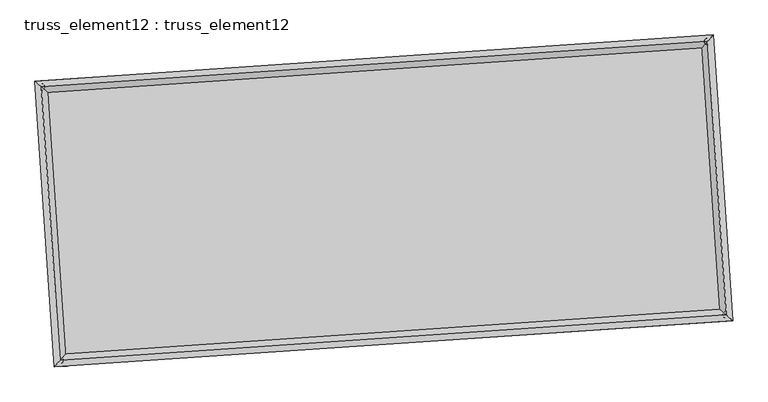
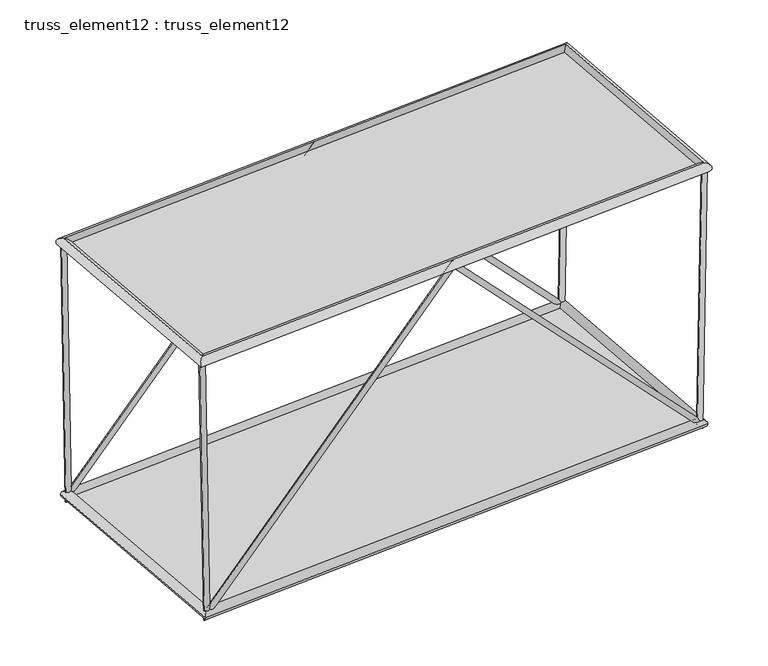
"""IFC4 building model written with IfcOpenShell, lengths in millimetres: plate geometry, truss_element12 : truss_element12."""

from ifc_helpers import new_model, si_unit, frame, origin, origin_with_axes, place, context, project, spatial, polyline, circle_curve, ellipse_curve, outline, extrude, source, transform, mapped, element, save
from ifc_brep_helpers import plane_surface, cylinder_surface, advanced_brep


def truss_element12_truss_element12_eb7cdb9d(model_context):
    return source(origin(), model_context, "Body", "SolidModel", [
        advanced_brep(
        [(-3751.912515, 2270.2937696, 5000.1099238), (-3851.0007491, 2256.9335317, 4998.3704092), (-3667.056332, 2276.0797902, 121.9949924), (-3761.9305509, 2263.0068899, -121.9949924), (1063.0047993, 2598.6046781, 5071.3707935), (1063.4636729, 2592.032179, 4927.1341285), (5794.4609613, 2921.2246878, 122.0048162), (5890.3000157, 2921.1558007, -122.0048162), (5877.9325391, 2926.9162974, 5000.120325), (5977.9176694, 2927.1301154, 4998.409186)],
        [
            (0, 1, circle_curve(frame((-3801.4566321, 2263.6136507, 4999.2401665), z_axis=(-0.017392638132463133, -0.0011859378786482353, 0.9998480332981313), x_axis=(-0.13360270549459097, 0.9910343071078557, -0.0011485729311865587)), 50.0)),
            (1, 0, circle_curve(frame((-3801.4566321, 2263.6136507, 4999.2401665), z_axis=(-0.017392638132463133, -0.0011859378786482353, 0.9998480332981313), x_axis=(-0.13360270549459097, 0.9910343071078557, -0.0011485729311865587)), 50.0)),
            (0, 2),
            (2, 3, ellipse_curve(frame((-3714.4934414, 2269.54334, 0.0), z_axis=(-0.9289957394028403, -0.06334468802646137, 0.36462908094418417), x_axis=(0.36378437978405503, 0.024805073983579777, 0.9311528517541036)), 131.300287, 50.0)),
            (3, 1),
            (3, 2, ellipse_curve(frame((-3714.4934414, 2269.54334, 0.0), z_axis=(-0.9289957394028403, -0.06334468802646137, 0.36462908094418417), x_axis=(0.36378437978405503, 0.024805073983579777, 0.9311528517541036)), 131.300287, 50.0)),
            (2, 4),
            (4, 5, ellipse_curve(frame((1063.2342361, 2595.3184285, 4999.252461), z_axis=(-0.9976833933321773, -0.06802823804168447, -7.414941499554083e-05), x_axis=(7.397764016911895e-05, 5.044254070666447e-06, -0.9999999972509321)), 72.2753704, 50.0)),
            (5, 3),
            (5, 4, ellipse_curve(frame((1063.2342361, 2595.3184285, 4999.252461), z_axis=(-0.9976833933321773, -0.06802823804168447, -7.414941499554083e-05), x_axis=(7.397764016911895e-05, 5.044254070666447e-06, -0.9999999972509321)), 72.2753704, 50.0)),
            (4, 6),
            (6, 7, ellipse_curve(frame((5842.3804885, 2921.1902443, 0.0), z_axis=(-0.9289170101606304, -0.06333931977871081, -0.36483053436384116), x_axis=(-0.36398536651592867, -0.02481877850480949, 0.9310739397039283)), 131.3219892, 50.0)),
            (7, 5),
            (7, 6, ellipse_curve(frame((5842.3804885, 2921.1902443, 0.0), z_axis=(-0.9289170101606304, -0.06333931977871081, -0.36483053436384116), x_axis=(-0.36398536651592867, -0.02481877850480949, 0.9310739397039283)), 131.3219892, 50.0)),
            (8, 9, circle_curve(frame((5927.9251043, 2927.0232064, 4999.2647555), z_axis=(0.017108923152044243, 0.001166592432629323, 0.9998529510936464), x_axis=(-0.002157828250047212, 0.9999970336184036, -0.001129836995660202)), 50.0)),
            (9, 8, circle_curve(frame((5927.9251043, 2927.0232064, 4999.2647555), z_axis=(0.017108923152044243, 0.001166592432629323, 0.9998529510936464), x_axis=(-0.002157828250047212, 0.9999970336184036, -0.001129836995660202)), 50.0)),
            (6, 8),
            (9, 7),
        ],
        [
            plane_surface(frame((-3801.4566321, 2313.6136155, 4999.2994724), z_axis=(-0.017392638132462068, -0.0011859378786532565, 0.9998480332981314), x_axis=(0.9998487366290929, -2.0629708890496073e-05, 0.017392625897830513))),
            cylinder_surface(frame((-3801.4566321, 2263.6136507, 4999.2401665), z_axis=(-0.017392638132463136, -0.0011859378786482355, 0.9998480332981315), x_axis=(-0.13360270549459097, 0.9910343071078557, -0.0011485729311865587)), 50.0),
            cylinder_surface(frame((-3714.4934414, 2269.54334, 0.0), z_axis=(-0.6901425550207472, -0.04705819734940098, -0.7221418003492527), x_axis=(-0.020412411512224723, 0.9987523229779233, -0.045575550489902014)), 50.0),
            cylinder_surface(frame((1063.2342361, 2595.3184285, 4999.252461), z_axis=(-0.6902493921239737, -0.047065482165348276, 0.7220392074264583), x_axis=(-0.11534170182495504, 0.9922794555315144, -0.045582605785589675)), 50.0),
            plane_surface(frame((5927.9251043, 2877.0232404, 4999.3230936), z_axis=(0.017108923152043723, 0.0011665924326239086, 0.9998529510936466), x_axis=(0.9998536316624437, -1.9962062093981113e-05, -0.017108911506539936))),
            cylinder_surface(frame((5842.3804885, 2921.1902443, 0.0), z_axis=(-0.017108923152044243, -0.001166592432629323, -0.9998529510936464), x_axis=(-0.002157828250047212, 0.9999970336184036, -0.001129836995660202)), 50.0),
        ],
        [
            (0, [[1, 2]]),
            (1, [[-1, 3, 4, 5]]),
            (1, [[-2, -5, 6, -3]]),
            (2, [[-4, 7, 8, 9]]),
            (2, [[-6, -9, 10, -7]]),
            (3, [[-8, 11, 12, 13]]),
            (3, [[-10, -13, 14, -11]]),
            (4, [[15, 16]]),
            (5, [[-12, 17, -16, 18]]),
            (5, [[-14, -18, -15, -17]]),
        ],
    ),
        advanced_brep(
        [(-3479.7995621, -1720.4398147, 5000.1099238), (-3578.8877962, -1733.8000526, 4998.3704092), (-3394.943379, -1714.6537941, 121.9949924), (-3489.817598, -1727.7266944, -121.9949924), (1335.1177522, -1392.1289062, 5071.3707935), (1335.5766258, -1398.7014053, 4927.1341285), (6066.5739142, -1069.5088965, 122.0048162), (6162.4129686, -1069.5777836, -122.0048162), (6150.045492, -1063.8172869, 5000.120325), (6250.0306223, -1063.6034689, 4998.409186)],
        [
            (0, 1, circle_curve(frame((-3529.3436792, -1727.1199336, 4999.2401665), z_axis=(-0.017392638132463636, -0.0011859378786482945, 0.9998480332981314), x_axis=(-0.1336027054945913, 0.9910343071078556, -0.0011485729311865723)), 50.0)),
            (1, 0, circle_curve(frame((-3529.3436792, -1727.1199336, 4999.2401665), z_axis=(-0.017392638132463636, -0.0011859378786482945, 0.9998480332981314), x_axis=(-0.1336027054945913, 0.9910343071078556, -0.0011485729311865723)), 50.0)),
            (0, 2),
            (2, 3, ellipse_curve(frame((-3442.3804885, -1721.1902443, 0.0), z_axis=(-0.9289957394028405, -0.06334468802646162, 0.3646290809441836), x_axis=(0.3637843797840544, 0.0248050739835798, 0.9311528517541038)), 131.300287, 50.0)),
            (3, 1),
            (3, 2, ellipse_curve(frame((-3442.3804885, -1721.1902443, 0.0), z_axis=(-0.9289957394028405, -0.06334468802646162, 0.3646290809441836), x_axis=(0.3637843797840544, 0.0248050739835798, 0.9311528517541038)), 131.300287, 50.0)),
            (2, 4),
            (4, 5, ellipse_curve(frame((1335.347189, -1395.4151558, 4999.252461), z_axis=(-0.9976833933321773, -0.06802823804168467, -7.414941499586186e-05), x_axis=(7.39776401694264e-05, 5.044254070676052e-06, -0.999999997250932)), 72.2753704, 50.0)),
            (5, 3),
            (5, 4, ellipse_curve(frame((1335.347189, -1395.4151558, 4999.252461), z_axis=(-0.9976833933321773, -0.06802823804168467, -7.414941499586186e-05), x_axis=(7.39776401694264e-05, 5.044254070676052e-06, -0.999999997250932)), 72.2753704, 50.0)),
            (4, 6),
            (6, 7, ellipse_curve(frame((6114.4934414, -1069.54334, 0.0), z_axis=(-0.9289170101606302, -0.063339319778711, -0.3648305343638408), x_axis=(-0.36398536651592855, -0.02481877850480956, 0.9310739397039284)), 131.3219892, 50.0)),
            (7, 5),
            (7, 6, ellipse_curve(frame((6114.4934414, -1069.54334, 0.0), z_axis=(-0.9289170101606302, -0.063339319778711, -0.3648305343638408), x_axis=(-0.36398536651592855, -0.02481877850480956, 0.9310739397039284)), 131.3219892, 50.0)),
            (8, 9, circle_curve(frame((6200.0380572, -1063.7103779, 4999.2647555), z_axis=(0.017108923152044368, 0.0011665924326293448, 0.9998529510936464), x_axis=(-0.0021578282500472473, 0.9999970336184036, -0.001129836995660223)), 50.0)),
            (9, 8, circle_curve(frame((6200.0380572, -1063.7103779, 4999.2647555), z_axis=(0.017108923152044368, 0.0011665924326293448, 0.9998529510936464), x_axis=(-0.0021578282500472473, 0.9999970336184036, -0.001129836995660223)), 50.0)),
            (6, 8),
            (9, 7),
        ],
        [
            plane_surface(frame((-3529.3436792, -1677.1199688, 4999.2994724), z_axis=(-0.017392638132462095, -0.0011859378786532565, 0.9998480332981314), x_axis=(0.9998487366290929, -2.0629708890496107e-05, 0.01739262589783054))),
            cylinder_surface(frame((-3529.3436792, -1727.1199336, 4999.2401665), z_axis=(-0.017392638132463636, -0.0011859378786482945, 0.9998480332981314), x_axis=(-0.1336027054945913, 0.9910343071078556, -0.0011485729311865723)), 50.0),
            cylinder_surface(frame((-3442.3804885, -1721.1902443, 0.0), z_axis=(-0.6901425550207463, -0.047058197349401074, -0.7221418003492535), x_axis=(-0.02041241151222477, 0.9987523229779234, -0.04557555048990207)), 50.0),
            cylinder_surface(frame((1335.347189, -1395.4151558, 4999.252461), z_axis=(-0.6902493921239734, -0.0470654821653484, 0.7220392074264587), x_axis=(-0.11534170182495534, 0.9922794555315144, -0.045582605785589723)), 50.0),
            plane_surface(frame((6200.0380572, -1113.7103439, 4999.3230936), z_axis=(0.017108923152043723, 0.0011665924326347361, 0.9998529510936466), x_axis=(0.9998536316624437, -1.9962062093537024e-05, -0.017108911506539936))),
            cylinder_surface(frame((6114.4934414, -1069.54334, 0.0), z_axis=(-0.017108923152044368, -0.0011665924326293448, -0.9998529510936464), x_axis=(-0.0021578282500472473, 0.9999970336184036, -0.001129836995660223)), 50.0),
        ],
        [
            (0, [[1, 2]]),
            (1, [[-1, 3, 4, 5]]),
            (1, [[-2, -5, 6, -3]]),
            (2, [[-4, 7, 8, 9]]),
            (2, [[-6, -9, 10, -7]]),
            (3, [[-8, 11, 12, 13]]),
            (3, [[-10, -13, 14, -11]]),
            (4, [[15, 16]]),
            (5, [[-12, 17, -16, 18]]),
            (5, [[-14, -18, -15, -17]]),
        ],
    ),
        advanced_brep(
        [(-3529.3372576, -1727.1128164, 4909.2401668), (-3529.3501007, -1727.1270509, 5089.2401662), (-3801.4639603, 2263.6198303, 5089.2401662), (-3801.4493039, 2263.607471, 4909.2401668), (5927.931073, 2927.0302928, 5089.2647552), (5927.9191355, 2927.0161201, 4909.2647557), (6200.0449326, -1063.7165884, 5089.2647552), (6200.0311818, -1063.7041673, 4909.2647557)],
        [
            (0, 1, ellipse_curve(frame((-3529.3436792, -1727.1199336, 4999.2401665), z_axis=(-0.7535719234032147, 0.6573654662782344, -1.782924587316493e-06), x_axis=(-0.657365466275839, -0.7535719234053045, -1.782924587316546e-06)), 127.2792206, 90.0)),
            (1, 2),
            (2, 3, ellipse_curve(frame((-3801.4566321, 2263.6136507, 4999.2401665), z_axis=(-0.6573654662758391, -0.7535719234053043, -1.7829245873165833e-06), x_axis=(0.7535719234032147, -0.6573654662782346, 1.7829245873165301e-06)), 127.2792206, 90.0)),
            (3, 0),
            (1, 0, ellipse_curve(frame((-3529.3436792, -1727.1199336, 4999.2401665), z_axis=(-0.7535719234032147, 0.6573654662782344, -1.782924587316493e-06), x_axis=(-0.657365466275839, -0.7535719234053045, -1.782924587316546e-06)), 127.2792206, 90.0)),
            (3, 2, ellipse_curve(frame((-3801.4566321, 2263.6136507, 4999.2401665), z_axis=(-0.6573654662758391, -0.7535719234053043, -1.7829245873165833e-06), x_axis=(0.7535719234032147, -0.6573654662782346, 1.7829245873165301e-06)), 127.2792206, 90.0)),
            (2, 4),
            (4, 5, ellipse_curve(frame((5927.9251043, 2927.0232064, 4999.2647555), z_axis=(-0.7535719234032134, 0.6573654662782359, -1.7829245873165754e-06), x_axis=(-0.6573654662758406, -0.7535719234053031, -1.782924587316538e-06)), 127.2792206, 90.0)),
            (5, 3),
            (5, 4, ellipse_curve(frame((5927.9251043, 2927.0232064, 4999.2647555), z_axis=(-0.7535719234032134, 0.6573654662782359, -1.7829245873165754e-06), x_axis=(-0.6573654662758406, -0.7535719234053031, -1.782924587316538e-06)), 127.2792206, 90.0)),
            (4, 6),
            (6, 7, ellipse_curve(frame((6200.0380572, -1063.7103779, 4999.2647555), z_axis=(0.6573654662758404, 0.753571923405303, 1.7829245873165003e-06), x_axis=(-0.7535719234032132, 0.6573654662782362, -1.7829245873165377e-06)), 127.2792206, 90.0)),
            (7, 5),
            (7, 6, ellipse_curve(frame((6200.0380572, -1063.7103779, 4999.2647555), z_axis=(0.6573654662758404, 0.753571923405303, 1.7829245873165003e-06), x_axis=(-0.7535719234032132, 0.6573654662782362, -1.7829245873165377e-06)), 127.2792206, 90.0)),
            (6, 1),
            (0, 7),
        ],
        [
            cylinder_surface(frame((-3529.3436792, -1727.1199336, 4999.2401665), z_axis=(0.0680282382287023, -0.9976833960748765, 0.0), x_axis=(-0.997683393150592, -0.06802823802930645, -7.656467492633377e-05)), 90.0),
            cylinder_surface(frame((-3801.4566321, 2263.6136507, 4999.2401665), z_axis=(-0.9976833960717054, -0.06802823822848186, -2.521436132071528e-06), x_axis=(-0.06802823785595627, 0.997683393352727, -7.404323880117403e-05)), 90.0),
            cylinder_surface(frame((5927.9251043, 2927.0232064, 4999.2647555), z_axis=(-0.06802823822869845, 0.9976833960748769, 0.0), x_axis=(0.9976833935231179, 0.0680282380547037, -7.152180267601429e-05)), 90.0),
            cylinder_surface(frame((6200.0380572, -1063.7103779, 4999.2647555), z_axis=(0.9976833960717054, 0.06802823822848189, 2.5214361320714755e-06), x_axis=(0.06802823822848189, -0.9976833933273259, -7.404323880117403e-05)), 90.0),
        ],
        [
            (0, [[1, 2, 3, 4]]),
            (0, [[5, -4, 6, -2]]),
            (1, [[-3, 7, 8, 9]]),
            (1, [[-6, -9, 10, -7]]),
            (2, [[-8, 11, 12, 13]]),
            (2, [[-10, -13, 14, -11]]),
            (3, [[-12, 15, -1, 16]]),
            (3, [[-14, -16, -5, -15]]),
        ],
    ),
        advanced_brep(
        [(-3358.7115243, -1625.2761972, 0.0), (-3526.0494527, -1817.1042913, 0.0), (-3810.4074885, 2353.2123043, 0.0), (-3618.5793943, 2185.8743758, 0.0), (5926.0494527, 3017.1042913, 0.0), (5758.7115243, 2825.2761972, 0.0), (6210.4074885, -1153.2123043, 0.0), (6018.5793943, -985.8743758, 0.0)],
        [
            (0, 1, ellipse_curve(frame((-3442.3804885, -1721.1902443, 0.0), z_axis=(-0.7535719234054579, 0.657365466278081, 0.0), x_axis=(-0.6573654662780811, -0.7535719234054578, 0.0)), 127.2792206, 90.0)),
            (1, 2),
            (2, 3, ellipse_curve(frame((-3714.4934414, 2269.54334, 0.0), z_axis=(-0.6573654662780811, -0.7535719234054578, 0.0), x_axis=(0.7535719234054579, -0.6573654662780809, 0.0)), 127.2792206, 90.0)),
            (3, 0),
            (1, 0, ellipse_curve(frame((-3442.3804885, -1721.1902443, 0.0), z_axis=(-0.7535719234054579, 0.657365466278081, 0.0), x_axis=(-0.6573654662780811, -0.7535719234054578, 0.0)), 127.2792206, 90.0)),
            (3, 2, ellipse_curve(frame((-3714.4934414, 2269.54334, 0.0), z_axis=(-0.6573654662780811, -0.7535719234054578, 0.0), x_axis=(0.7535719234054579, -0.6573654662780809, 0.0)), 127.2792206, 90.0)),
            (2, 4),
            (4, 5, ellipse_curve(frame((5842.3804885, 2921.1902443, 0.0), z_axis=(-0.7535719234054563, 0.6573654662780827, 0.0), x_axis=(-0.6573654662780828, -0.7535719234054563, 0.0)), 127.2792206, 90.0)),
            (5, 3),
            (5, 4, ellipse_curve(frame((5842.3804885, 2921.1902443, 0.0), z_axis=(-0.7535719234054563, 0.6573654662780827, 0.0), x_axis=(-0.6573654662780828, -0.7535719234054563, 0.0)), 127.2792206, 90.0)),
            (4, 6),
            (6, 7, ellipse_curve(frame((6114.4934414, -1069.54334, 0.0), z_axis=(0.6573654662780827, 0.7535719234054564, 0.0), x_axis=(-0.7535719234054565, 0.6573654662780825, 0.0)), 127.2792206, 90.0)),
            (7, 5),
            (7, 6, ellipse_curve(frame((6114.4934414, -1069.54334, 0.0), z_axis=(0.6573654662780827, 0.7535719234054564, 0.0), x_axis=(-0.7535719234054565, 0.6573654662780825, 0.0)), 127.2792206, 90.0)),
            (6, 1),
            (0, 7),
        ],
        [
            cylinder_surface(frame((-3442.3804885, -1721.1902443, 0.0), z_axis=(0.06802823822870294, -0.9976833960748764, 0.0), x_axis=(-0.9976833960748764, -0.06802823822870294, 0.0)), 90.0),
            cylinder_surface(frame((-3714.4934414, 2269.54334, 0.0), z_axis=(-0.9976833960748768, -0.06802823822869876, 0.0), x_axis=(-0.06802823822869876, 0.9976833960748768, 0.0)), 90.0),
            cylinder_surface(frame((5842.3804885, 2921.1902443, 0.0), z_axis=(-0.06802823822869875, 0.9976833960748768, 0.0), x_axis=(0.9976833960748768, 0.06802823822869875, 0.0)), 90.0),
            cylinder_surface(frame((6114.4934414, -1069.54334, 0.0), z_axis=(0.9976833960748768, 0.06802823822869897, 0.0), x_axis=(0.06802823822869897, -0.9976833960748768, 0.0)), 90.0),
        ],
        [
            (0, [[1, 2, 3, 4]]),
            (0, [[5, -4, 6, -2]]),
            (1, [[-3, 7, 8, 9]]),
            (1, [[-6, -9, 10, -7]]),
            (2, [[-8, 11, 12, 13]]),
            (2, [[-10, -13, 14, -11]]),
            (3, [[-12, 15, -1, 16]]),
            (3, [[-14, -16, -5, -15]]),
        ],
    ),
        extrude(outline(polyline([(-3442.3804885, -1721.1902443), (-3714.4934414, 2269.54334), (5842.3804885, 2921.1902443), (6114.4934414, -1069.54334), (-3442.3804885, -1721.1902443)])), origin_with_axes(), (0.0, 0.0, 1.0), 20.0),
        extrude(outline(polyline([(-2000.0, 4875.9865979), (2000.0, 4875.9865978), (2000.0, -4875.986598), (-2000.0, -4875.9865979), (-2000.0, 4875.9865979)])), frame((1199.2907125, 599.9516364, 4999.252461), z_axis=(-2.5155949632309937e-06, -1.7152885787101881e-07, 0.9999999999968213), x_axis=(-0.06802823822870278, 0.9976833960748764, 0.0)), (0.0, 0.0, 1.0), 20.0),
    ])


if __name__ == "__main__":
    model = new_model("IFC4")
    model_context = context("Model", 3, world=origin())
    ifc_project = project(units=[si_unit("LENGTHUNIT", "METRE", prefix="MILLI")], contexts=[model_context])
    site = spatial("IfcSite", under=ifc_project)
    building = spatial("IfcBuilding", under=site)
    placement = place(None, origin())
    truss_element12_truss_element12_shape = truss_element12_truss_element12_eb7cdb9d(model_context)
    element("IfcPlate", 1, ObjectType="truss_element12 : truss_element12", at=placement, inside=building, context=model_context, shape_type="MappedRepresentation", body=[
        mapped(truss_element12_truss_element12_shape, transform((0.0, 0.0, 0.0), x_axis=(1.0, 0.0, 0.0), y_axis=(0.0, 1.0, 0.0), z_axis=(0.0, 0.0, 1.0))),
    ])
    save(model, "model.ifc")

# Revit data of these elements
# Type "truss_element12 : truss_element12"
#   steellbar1 = 90 mm
#   steelbar2 = 50 mm
#   offset1 = 5000 mm
#   M = Default Roof
# Element 1 (IfcPlate, "truss_element12 : truss_element12")
#   Materials on its faces: "Default Roof"
# Materials
#   "Default Roof": class "Miscellaneous", colour RGB 0 127 0, transparency 0, Comments = "Rendering appearance not upgraded Rendering appearance not upgraded ", Cost = 0
